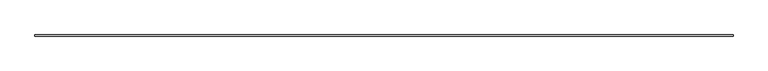
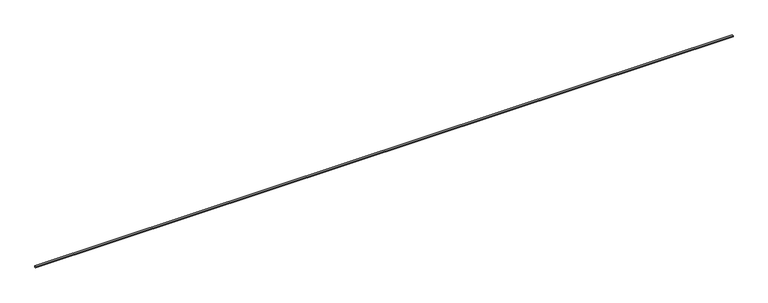
"""IFC4 building model written with IfcOpenShell, lengths in millimetres: proxy geometry, Joint002 1693 : Joint002 1693."""

from ifc_helpers import new_model, si_unit, point, frame, frame_2d, origin, place, context, project, spatial, polyline, circle_curve, trimmed, segment, composite_curve, outline, extrude, source, transform, mapped, element, save


def generic_models_1a41533e(model_context):
    return source(origin(), model_context, "Body", "SweptSolid", [
        extrude(outline(composite_curve([segment(polyline([(9718.4918386, 37509.421875), (9718.4918386, 37513.3398437)]), True, "CONTINUOUS"), segment(trimmed(circle_curve(frame_2d((9720.0901706, 37518.5117187)), 5.4132205), [point((9718.4918386, 37513.3398437))], [point((9721.6885026, 37513.3398437))], True, "CARTESIAN"), True, "CONTINUOUS"), segment(polyline([(9721.6885026, 37513.3398437), (9721.6885026, 37509.421875)]), True, "CONTINUOUS"), segment(trimmed(circle_curve(frame_2d((9720.0901706, 37514.59375)), 5.4132205), [point((9721.6885026, 37509.421875))], [point((9718.4918386, 37509.421875))], False, "CARTESIAN"), True, "CONTINUOUS")], self_intersect=False)), frame((3694.2883192, 0.0, 0.0), z_axis=(1.0, 0.0, 0.0), x_axis=(0.0, 1.0, 0.0)), (0.0, 0.0, 1.0), 2000.0),
    ])


if __name__ == "__main__":
    model = new_model("IFC4")
    model_context = context("Model", 3, world=origin())
    ifc_project = project(units=[si_unit("LENGTHUNIT", "METRE", prefix="MILLI")], contexts=[model_context])
    site = spatial("IfcSite", under=ifc_project)
    building = spatial("IfcBuilding", under=site)
    placement = place(None, origin())
    generic_models_shape = generic_models_1a41533e(model_context)
    element("IfcBuildingElementProxy", 1, Name="Joint002 1693 : Joint002 1693", ObjectType="Joint002 1693 : Joint002 1693", at=placement, inside=building, context=model_context, shape_type="MappedRepresentation", body=[
        mapped(generic_models_shape, transform((0.0, 0.0, 0.0), x_axis=(1.0, 0.0, 0.0), y_axis=(0.0, 1.0, 0.0), z_axis=(0.0, 0.0, 1.0))),
    ])
    save(model, "model.ifc")

# Revit data of these elements
# Type "Joint002 1693 : Joint002 1693"
#   NameOverride = "Joint002"
# Element 1 (IfcBuildingElementProxy, "Joint002 1693 : Joint002 1693")
#   Materials on its faces: "SILICON JOINT"
# Materials
#   "SILICON JOINT": class "Unassigned", colour RGB 150 184 127, transparency 0
